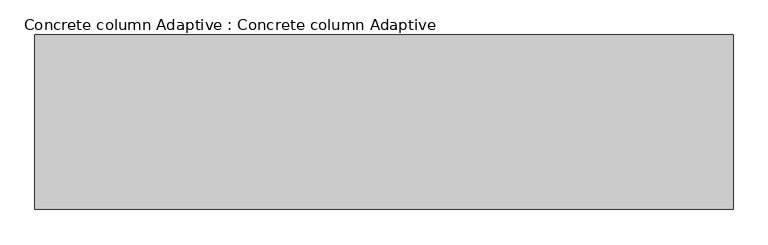
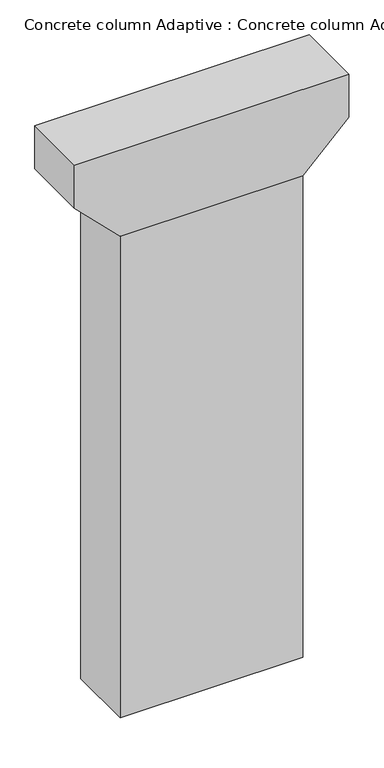
"""IFC4 building model written with IfcOpenShell, lengths in millimetres: proxy geometry, Concrete column Adaptive : Concrete column Adaptive."""

import ifcopenshell
import ifcopenshell.guid

model = None  # the IFC model being written
_history = None  # IfcOwnerHistory: only IFC2X3 demands one
_inside = {}  # id of a spatial element -> (the spatial element, [elements in it])
_under = {}  # id of a project, library or spatial element -> (it, [spatial elements below it])
_declared = {}  # id of a project -> (the project, [libraries it declares])
_typed = {}  # id of a type object -> (the type object, [elements of that type])
_made_of = {}  # id of a material, layer set ... -> (it, [elements and type objects made of it])


def new_model(schema):
    """Start an empty IFC model of exactly this schema.

    Asked for "IFC4X3", IfcOpenShell would pick the latest addendum, in which some entities
    have other attributes; the version numbers below select the first issue.
    IFC2X3 requires an IfcOwnerHistory on every rooted entity: one is made here for all.
    """
    global model, _history
    if schema == "IFC4X3":
        model = ifcopenshell.file(schema_version=(4, 3, 0, 0))
    else:
        model = ifcopenshell.file(schema=schema)
    _inside.clear()
    _under.clear()
    _declared.clear()
    _typed.clear()
    _made_of.clear()
    _history = None
    if model.schema == "IFC2X3":
        org = make("IfcOrganization", Name="unknown")
        user = make(
            "IfcPersonAndOrganization",
            ThePerson=make("IfcPerson", FamilyName="unknown"),
            TheOrganization=org,
        )
        app = make(
            "IfcApplication",
            ApplicationDeveloper=org,
            Version="unknown",
            ApplicationFullName="unknown",
            ApplicationIdentifier="unknown",
        )
        _history = make(
            "IfcOwnerHistory",
            OwningUser=user,
            OwningApplication=app,
            ChangeAction="ADDED",
            CreationDate=0,
        )
    return model


def make(cls, **values):
    """One entity of the class cls with the attributes given. An attribute that is None is left unset."""
    return model.create_entity(
        cls, **{name: value for name, value in values.items() if value is not None}
    )


def rooted(cls, **values):
    """An entity with a GlobalId (a new one), such as an element, a storey or a relation."""
    return make(cls, GlobalId=ifcopenshell.guid.new(), OwnerHistory=_history, **values)


def si_unit(unit_type, name, prefix=None):
    """IfcSIUnit, for example si_unit("LENGTHUNIT", "METRE", prefix="MILLI")."""
    return make("IfcSIUnit", UnitType=unit_type, Prefix=prefix, Name=name)


def assignment(units):
    """IfcUnitAssignment: the units of a project."""
    return None if units is None else make("IfcUnitAssignment", Units=units)


def point(xyz):
    """IfcCartesianPoint."""
    return None if xyz is None else make("IfcCartesianPoint", Coordinates=xyz)


def direction(xyz):
    """IfcDirection."""
    return None if xyz is None else make("IfcDirection", DirectionRatios=xyz)


def frame(location, z_axis=None, x_axis=None):
    """IfcAxis2Placement3D, a coordinate frame: its origin and axes. An axis left out is left unset."""
    return make(
        "IfcAxis2Placement3D",
        Location=point(location),
        Axis=direction(z_axis),
        RefDirection=direction(x_axis),
    )


def origin():
    """The frame at (0, 0, 0) with its axes left unset."""
    return frame((0.0, 0.0, 0.0))


def origin_with_axes():
    """The frame at (0, 0, 0) with the z axis (0, 0, 1) and the x axis (1, 0, 0) written out."""
    return frame((0.0, 0.0, 0.0), z_axis=(0.0, 0.0, 1.0), x_axis=(1.0, 0.0, 0.0))


def place(relative_to, where):
    """IfcLocalPlacement: puts the frame where relative to a parent placement (None: the world)."""
    return make(
        "IfcLocalPlacement", PlacementRelTo=relative_to, RelativePlacement=where
    )


def context(
    kind, dimensions, precision=None, world=None, true_north=None, identifier=None
):
    """IfcGeometricRepresentationContext, for example the 3D "Model" context."""
    return make(
        "IfcGeometricRepresentationContext",
        ContextIdentifier=identifier,
        ContextType=kind,
        CoordinateSpaceDimension=dimensions,
        Precision=precision,
        WorldCoordinateSystem=world,
        TrueNorth=true_north,
    )


def project(units=None, contexts=None):
    """IfcProject with its units and contexts."""
    return rooted(
        "IfcProject",
        Name="project",
        RepresentationContexts=contexts,
        UnitsInContext=assignment(units),
    )


def spatial(cls, under=None, at=None, **own):
    """A site, building, storey or space (cls), placed at a placement, below another one or the project."""
    s = rooted(cls, ObjectPlacement=at, **own)
    if under is not None:
        _under.setdefault(under.id(), (under, []))[1].append(s)
    return s


def polyline(points):
    """IfcPolyline through the points."""
    return make("IfcPolyline", Points=[point(p) for p in points])


def outline(outer, holes=None, kind="AREA"):
    """IfcArbitraryClosedProfileDef: a profile drawn as a closed curve; with holes, ...WithVoids."""
    if holes is None:
        return make("IfcArbitraryClosedProfileDef", ProfileType=kind, OuterCurve=outer)
    return make(
        "IfcArbitraryProfileDefWithVoids",
        ProfileType=kind,
        OuterCurve=outer,
        InnerCurves=holes,
    )


def extrude(swept, where, along, depth):
    """IfcExtrudedAreaSolid: the profile swept, set in the frame where, extruded along a direction by depth."""
    return make(
        "IfcExtrudedAreaSolid",
        SweptArea=swept,
        Position=where,
        ExtrudedDirection=direction(along),
        Depth=depth,
    )


def shape(context_of_items, identifier, shape_type, items):
    """IfcShapeRepresentation: the items that make up one representation, for example the "Body"."""
    return make(
        "IfcShapeRepresentation",
        ContextOfItems=context_of_items,
        RepresentationIdentifier=identifier,
        RepresentationType=shape_type,
        Items=items,
    )


def source(mapping_origin, context_of_items, identifier, shape_type, items):
    """IfcRepresentationMap: a shape defined once, which mapped items show again and again."""
    return make(
        "IfcRepresentationMap",
        MappingOrigin=mapping_origin,
        MappedRepresentation=shape(context_of_items, identifier, shape_type, items),
    )


def transform(
    local_origin,
    x_axis=None,
    y_axis=None,
    z_axis=None,
    scale=None,
    scale2=None,
    scale3=None,
    uniform=True,
):
    """IfcCartesianTransformationOperator3D, or its non-uniform kind. x_axis, y_axis, z_axis: its Axis1, 2, 3."""
    if uniform:
        return make(
            "IfcCartesianTransformationOperator3D",
            Axis1=direction(x_axis),
            Axis2=direction(y_axis),
            LocalOrigin=point(local_origin),
            Scale=scale,
            Axis3=direction(z_axis),
        )
    return make(
        "IfcCartesianTransformationOperator3DnonUniform",
        Axis1=direction(x_axis),
        Axis2=direction(y_axis),
        LocalOrigin=point(local_origin),
        Scale=scale,
        Axis3=direction(z_axis),
        Scale2=scale2,
        Scale3=scale3,
    )


def mapped(mapping_source, mapping_target):
    """IfcMappedItem: shows the shape of a source again, moved by a transform."""
    return make(
        "IfcMappedItem", MappingSource=mapping_source, MappingTarget=mapping_target
    )


def made_of(thing, what):
    """Note that an element or type object is made of a material, layer set ...; save() writes the relation."""
    if what is not None:
        _made_of.setdefault(what.id(), (what, []))[1].append(thing)
    return thing


def element(
    cls,
    number,
    at=None,
    inside=None,
    cuts=None,
    type_object=None,
    material=None,
    context=None,
    identifier="Body",
    shape_type=None,
    held_by="IfcProductDefinitionShape",
    body=None,
    shapes=None,
    **own,
):
    """One element of the class cls, such as IfcWall. Its Tag is "e" and its number.

    at: its placement. inside: the storey or other place that contains it. cuts: it is an
    opening in that element (IfcRelVoidsElement). A single representation is given by context,
    identifier, shape_type and body (its items); several are given by shapes. held_by: the class
    of the entity that holds the representations. save() writes the other relations.
    """
    e = rooted(cls, Tag="e%d" % number, ObjectPlacement=at, **own)
    if body is not None:
        shapes = [shape(context, identifier, shape_type, body)]
    if shapes is not None:
        e.Representation = make(held_by, Representations=shapes)
    if inside is not None:
        _inside.setdefault(inside.id(), (inside, []))[1].append(e)
    if cuts is not None:
        rooted(
            "IfcRelVoidsElement", RelatingBuildingElement=cuts, RelatedOpeningElement=e
        )
    if type_object is not None:
        _typed.setdefault(type_object.id(), (type_object, []))[1].append(e)
    return made_of(e, material)


def aggregate(whole, parts):
    """IfcRelAggregates: a whole, such as a stair, and the parts it consists of."""
    return rooted("IfcRelAggregates", RelatingObject=whole, RelatedObjects=parts)


def save(model, path):
    """Write the relations noted so far, then the file.

    IfcRelAggregates (storeys below a building ...), IfcRelContainedInSpatialStructure (elements
    in a storey), IfcRelDefinesByType, IfcRelAssociatesMaterial and IfcRelDeclares: one each for
    every whole, place, type object, material and project.
    """
    for whole, parts in _under.values():
        aggregate(whole, parts)
    for where, things in _inside.values():
        rooted(
            "IfcRelContainedInSpatialStructure",
            RelatedElements=things,
            RelatingStructure=where,
        )
    for kind, things in _typed.values():
        rooted("IfcRelDefinesByType", RelatedObjects=things, RelatingType=kind)
    for what, things in _made_of.values():
        rooted("IfcRelAssociatesMaterial", RelatedObjects=things, RelatingMaterial=what)
    for by, libraries in _declared.values():
        rooted("IfcRelDeclares", RelatingContext=by, RelatedDefinitions=libraries)
    model.write(path)


def concrete_column_adaptive_concrete_column_adaptive_6c7a738b(model_context):
    return source(origin(), model_context, "Body", "SweptSolid", [
        extrude(outline(polyline([(26284.0, 6000.0), (26284.0, -6000.0), (24284.0, -6000.0), (22284.0, -4000.0), (22284.0, 4000.0), (24284.0, 6000.0), (26284.0, 6000.0)])), frame((0.0, -1500.0, 0.0), z_axis=(0.0, 1.0, 0.0), x_axis=(0.0, 0.0, 1.0)), (0.0, 0.0, 1.0), 3000.0),
        extrude(outline(polyline([(-4000.0, -1500.0), (-4000.0, 1500.0), (4000.0, 1500.0), (4000.0, -1500.0), (-4000.0, -1500.0)])), origin_with_axes(), (0.0, 0.0, 1.0), 22284.0),
    ])


if __name__ == "__main__":
    model = new_model("IFC4")
    model_context = context("Model", 3, world=origin())
    ifc_project = project(units=[si_unit("LENGTHUNIT", "METRE", prefix="MILLI")], contexts=[model_context])
    site = spatial("IfcSite", under=ifc_project)
    building = spatial("IfcBuilding", under=site)
    placement = place(None, origin())
    concrete_column_adaptive_concrete_column_adaptive_shape = concrete_column_adaptive_concrete_column_adaptive_6c7a738b(model_context)
    element("IfcBuildingElementProxy", 1, Name="Concrete column Adaptive : Concrete column Adaptive", ObjectType="Concrete column Adaptive : Concrete column Adaptive", at=placement, inside=building, context=model_context, shape_type="MappedRepresentation", body=[
        mapped(concrete_column_adaptive_concrete_column_adaptive_shape, transform((0.0, 0.0, 0.0), x_axis=(1.0, 0.0, 0.0), y_axis=(0.0, 1.0, 0.0), z_axis=(0.0, 0.0, 1.0))),
    ])
    save(model, "model.ifc")

# Revit data of these elements
# Type "Concrete column Adaptive : Concrete column Adaptive"
#   Height [instance default] = 30000 mm
#   Default Elevation = 0
# Element 1 (IfcBuildingElementProxy, "Concrete column Adaptive : Concrete column Adaptive")
#   Height = 22284 mm
